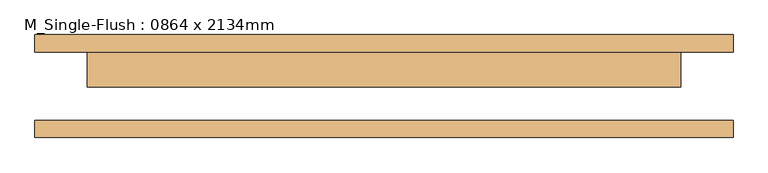
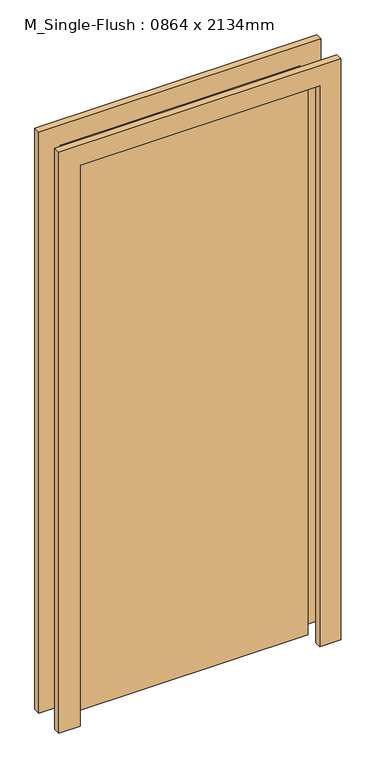
"""IFC4 building model written with IfcOpenShell, lengths in millimetres: door geometry, M_Single-Flush : 0864 x 2134mm."""

import ifcopenshell
import ifcopenshell.guid

model = None  # the IFC model being written
_history = None  # IfcOwnerHistory: only IFC2X3 demands one
_inside = {}  # id of a spatial element -> (the spatial element, [elements in it])
_under = {}  # id of a project, library or spatial element -> (it, [spatial elements below it])
_declared = {}  # id of a project -> (the project, [libraries it declares])
_typed = {}  # id of a type object -> (the type object, [elements of that type])
_made_of = {}  # id of a material, layer set ... -> (it, [elements and type objects made of it])


def new_model(schema):
    """Start an empty IFC model of exactly this schema.

    Asked for "IFC4X3", IfcOpenShell would pick the latest addendum, in which some entities
    have other attributes; the version numbers below select the first issue.
    IFC2X3 requires an IfcOwnerHistory on every rooted entity: one is made here for all.
    """
    global model, _history
    if schema == "IFC4X3":
        model = ifcopenshell.file(schema_version=(4, 3, 0, 0))
    else:
        model = ifcopenshell.file(schema=schema)
    _inside.clear()
    _under.clear()
    _declared.clear()
    _typed.clear()
    _made_of.clear()
    _history = None
    if model.schema == "IFC2X3":
        org = make("IfcOrganization", Name="unknown")
        user = make(
            "IfcPersonAndOrganization",
            ThePerson=make("IfcPerson", FamilyName="unknown"),
            TheOrganization=org,
        )
        app = make(
            "IfcApplication",
            ApplicationDeveloper=org,
            Version="unknown",
            ApplicationFullName="unknown",
            ApplicationIdentifier="unknown",
        )
        _history = make(
            "IfcOwnerHistory",
            OwningUser=user,
            OwningApplication=app,
            ChangeAction="ADDED",
            CreationDate=0,
        )
    return model


def make(cls, **values):
    """One entity of the class cls with the attributes given. An attribute that is None is left unset."""
    return model.create_entity(
        cls, **{name: value for name, value in values.items() if value is not None}
    )


def rooted(cls, **values):
    """An entity with a GlobalId (a new one), such as an element, a storey or a relation."""
    return make(cls, GlobalId=ifcopenshell.guid.new(), OwnerHistory=_history, **values)


def si_unit(unit_type, name, prefix=None):
    """IfcSIUnit, for example si_unit("LENGTHUNIT", "METRE", prefix="MILLI")."""
    return make("IfcSIUnit", UnitType=unit_type, Prefix=prefix, Name=name)


def assignment(units):
    """IfcUnitAssignment: the units of a project."""
    return None if units is None else make("IfcUnitAssignment", Units=units)


def point(xyz):
    """IfcCartesianPoint."""
    return None if xyz is None else make("IfcCartesianPoint", Coordinates=xyz)


def direction(xyz):
    """IfcDirection."""
    return None if xyz is None else make("IfcDirection", DirectionRatios=xyz)


def frame(location, z_axis=None, x_axis=None):
    """IfcAxis2Placement3D, a coordinate frame: its origin and axes. An axis left out is left unset."""
    return make(
        "IfcAxis2Placement3D",
        Location=point(location),
        Axis=direction(z_axis),
        RefDirection=direction(x_axis),
    )


def origin():
    """The frame at (0, 0, 0) with its axes left unset."""
    return frame((0.0, 0.0, 0.0))


def origin_with_axes():
    """The frame at (0, 0, 0) with the z axis (0, 0, 1) and the x axis (1, 0, 0) written out."""
    return frame((0.0, 0.0, 0.0), z_axis=(0.0, 0.0, 1.0), x_axis=(1.0, 0.0, 0.0))


def place(relative_to, where):
    """IfcLocalPlacement: puts the frame where relative to a parent placement (None: the world)."""
    return make(
        "IfcLocalPlacement", PlacementRelTo=relative_to, RelativePlacement=where
    )


def context(
    kind, dimensions, precision=None, world=None, true_north=None, identifier=None
):
    """IfcGeometricRepresentationContext, for example the 3D "Model" context."""
    return make(
        "IfcGeometricRepresentationContext",
        ContextIdentifier=identifier,
        ContextType=kind,
        CoordinateSpaceDimension=dimensions,
        Precision=precision,
        WorldCoordinateSystem=world,
        TrueNorth=true_north,
    )


def project(units=None, contexts=None):
    """IfcProject with its units and contexts."""
    return rooted(
        "IfcProject",
        Name="project",
        RepresentationContexts=contexts,
        UnitsInContext=assignment(units),
    )


def spatial(cls, under=None, at=None, **own):
    """A site, building, storey or space (cls), placed at a placement, below another one or the project."""
    s = rooted(cls, ObjectPlacement=at, **own)
    if under is not None:
        _under.setdefault(under.id(), (under, []))[1].append(s)
    return s


def polyline(points):
    """IfcPolyline through the points."""
    return make("IfcPolyline", Points=[point(p) for p in points])


def outline(outer, holes=None, kind="AREA"):
    """IfcArbitraryClosedProfileDef: a profile drawn as a closed curve; with holes, ...WithVoids."""
    if holes is None:
        return make("IfcArbitraryClosedProfileDef", ProfileType=kind, OuterCurve=outer)
    return make(
        "IfcArbitraryProfileDefWithVoids",
        ProfileType=kind,
        OuterCurve=outer,
        InnerCurves=holes,
    )


def extrude(swept, where, along, depth):
    """IfcExtrudedAreaSolid: the profile swept, set in the frame where, extruded along a direction by depth."""
    return make(
        "IfcExtrudedAreaSolid",
        SweptArea=swept,
        Position=where,
        ExtrudedDirection=direction(along),
        Depth=depth,
    )


def shape(context_of_items, identifier, shape_type, items):
    """IfcShapeRepresentation: the items that make up one representation, for example the "Body"."""
    return make(
        "IfcShapeRepresentation",
        ContextOfItems=context_of_items,
        RepresentationIdentifier=identifier,
        RepresentationType=shape_type,
        Items=items,
    )


def source(mapping_origin, context_of_items, identifier, shape_type, items):
    """IfcRepresentationMap: a shape defined once, which mapped items show again and again."""
    return make(
        "IfcRepresentationMap",
        MappingOrigin=mapping_origin,
        MappedRepresentation=shape(context_of_items, identifier, shape_type, items),
    )


def transform(
    local_origin,
    x_axis=None,
    y_axis=None,
    z_axis=None,
    scale=None,
    scale2=None,
    scale3=None,
    uniform=True,
):
    """IfcCartesianTransformationOperator3D, or its non-uniform kind. x_axis, y_axis, z_axis: its Axis1, 2, 3."""
    if uniform:
        return make(
            "IfcCartesianTransformationOperator3D",
            Axis1=direction(x_axis),
            Axis2=direction(y_axis),
            LocalOrigin=point(local_origin),
            Scale=scale,
            Axis3=direction(z_axis),
        )
    return make(
        "IfcCartesianTransformationOperator3DnonUniform",
        Axis1=direction(x_axis),
        Axis2=direction(y_axis),
        LocalOrigin=point(local_origin),
        Scale=scale,
        Axis3=direction(z_axis),
        Scale2=scale2,
        Scale3=scale3,
    )


def mapped(mapping_source, mapping_target):
    """IfcMappedItem: shows the shape of a source again, moved by a transform."""
    return make(
        "IfcMappedItem", MappingSource=mapping_source, MappingTarget=mapping_target
    )


def made_of(thing, what):
    """Note that an element or type object is made of a material, layer set ...; save() writes the relation."""
    if what is not None:
        _made_of.setdefault(what.id(), (what, []))[1].append(thing)
    return thing


def element(
    cls,
    number,
    at=None,
    inside=None,
    cuts=None,
    type_object=None,
    material=None,
    context=None,
    identifier="Body",
    shape_type=None,
    held_by="IfcProductDefinitionShape",
    body=None,
    shapes=None,
    **own,
):
    """One element of the class cls, such as IfcWall. Its Tag is "e" and its number.

    at: its placement. inside: the storey or other place that contains it. cuts: it is an
    opening in that element (IfcRelVoidsElement). A single representation is given by context,
    identifier, shape_type and body (its items); several are given by shapes. held_by: the class
    of the entity that holds the representations. save() writes the other relations.
    """
    e = rooted(cls, Tag="e%d" % number, ObjectPlacement=at, **own)
    if body is not None:
        shapes = [shape(context, identifier, shape_type, body)]
    if shapes is not None:
        e.Representation = make(held_by, Representations=shapes)
    if inside is not None:
        _inside.setdefault(inside.id(), (inside, []))[1].append(e)
    if cuts is not None:
        rooted(
            "IfcRelVoidsElement", RelatingBuildingElement=cuts, RelatedOpeningElement=e
        )
    if type_object is not None:
        _typed.setdefault(type_object.id(), (type_object, []))[1].append(e)
    return made_of(e, material)


def aggregate(whole, parts):
    """IfcRelAggregates: a whole, such as a stair, and the parts it consists of."""
    return rooted("IfcRelAggregates", RelatingObject=whole, RelatedObjects=parts)


def save(model, path):
    """Write the relations noted so far, then the file.

    IfcRelAggregates (storeys below a building ...), IfcRelContainedInSpatialStructure (elements
    in a storey), IfcRelDefinesByType, IfcRelAssociatesMaterial and IfcRelDeclares: one each for
    every whole, place, type object, material and project.
    """
    for whole, parts in _under.values():
        aggregate(whole, parts)
    for where, things in _inside.values():
        rooted(
            "IfcRelContainedInSpatialStructure",
            RelatedElements=things,
            RelatingStructure=where,
        )
    for kind, things in _typed.values():
        rooted("IfcRelDefinesByType", RelatedObjects=things, RelatingType=kind)
    for what, things in _made_of.values():
        rooted("IfcRelAssociatesMaterial", RelatedObjects=things, RelatingMaterial=what)
    for by, libraries in _declared.values():
        rooted("IfcRelDeclares", RelatingContext=by, RelatedDefinitions=libraries)
    model.write(path)


def m_single_flush_0864_x_2134mm_3838e64d(model_context):
    return source(origin(), model_context, "Body", "SweptSolid", [
        extrude(outline(polyline([(2210.0, -508.0), (0.0, -508.0), (0.0, -432.0), (2134.0, -432.0), (2134.0, 432.0), (0.0, 432.0), (0.0, 508.0), (2210.0, 508.0), (2210.0, -508.0)])), frame((0.0, 50.0, 0.0), z_axis=(0.0, 1.0, 0.0), x_axis=(0.0, 0.0, 1.0)), (0.0, 0.0, 1.0), 25.0),
        extrude(outline(polyline([(2210.0, 508.0), (2210.0, -508.0), (0.0, -508.0), (0.0, -432.0), (2134.0, -432.0), (2134.0, 432.0), (0.0, 432.0), (0.0, 508.0), (2210.0, 508.0)])), frame((0.0, -75.0, 0.0), z_axis=(0.0, 1.0, 0.0), x_axis=(0.0, 0.0, 1.0)), (0.0, 0.0, 1.0), 25.0),
        extrude(outline(polyline([(432.0, -1.0), (-432.0, -1.0), (-432.0, 50.0), (432.0, 50.0), (432.0, -1.0)])), origin_with_axes(), (0.0, 0.0, 1.0), 2134.0),
    ])


if __name__ == "__main__":
    model = new_model("IFC4")
    model_context = context("Model", 3, world=origin())
    ifc_project = project(units=[si_unit("LENGTHUNIT", "METRE", prefix="MILLI")], contexts=[model_context])
    site = spatial("IfcSite", under=ifc_project)
    building = spatial("IfcBuilding", under=site)
    placement = place(None, origin())
    m_single_flush_0864_x_2134mm_shape = m_single_flush_0864_x_2134mm_3838e64d(model_context)
    element("IfcDoor", 1, ObjectType="M_Single-Flush : 0864 x 2134mm", at=placement, inside=building, context=model_context, shape_type="MappedRepresentation", body=[
        mapped(m_single_flush_0864_x_2134mm_shape, transform((0.0, 0.0, 0.0), x_axis=(1.0, 0.0, 0.0), y_axis=(0.0, 1.0, 0.0), z_axis=(0.0, 0.0, 1.0))),
    ])
    save(model, "model.ifc")

# Revit data of these elements
# Project information
#   Organization Name = "SHV"
#   Building Name = "Pere Valencia"
#   Author = "Ian Salter"
#   Project Issue Date = "Issue Date"
#   Project Status = "Project  Status"
#   Client Name = "Ian Salter"
#   Project Address = "## Street\nCity, State  Zip"
#   Project Name = "Project Name"
#   Project Number = "Project  Number"
# Type "M_Single-Flush : 0864 x 2134mm"
#   Type Mark = "16"
#   Thickness = 5.1 cm
#   Height = 213.4 cm
#   Trim Projection Ext = 2.5 cm
#   Trim Projection Int = 2.5 cm
#   Trim Width = 7.6 cm
#   Width = 86.4 cm
#   Door Material = Door - Panel
#   Frame Material = Door - Frame
#   Function = (empty or 0)
#   Wall Closure = (empty or 0)
# Element 1 (IfcDoor, "M_Single-Flush : 0864 x 2134mm")
#   Materials on its faces: "Door - Frame", "Door - Panel"
# Materials
#   "Door - Panel": class "Wood", colour RGB 114 82 51, transparency 0
#   "Door - Frame": class "Miscellaneous", colour RGB 153 76 43, transparency 0
